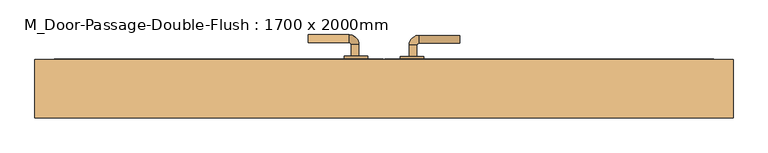
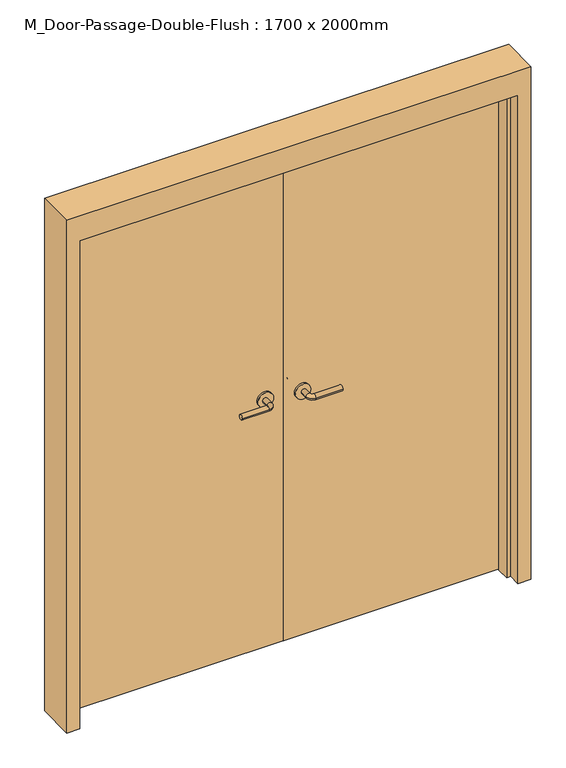
"""IFC4 building model written with IfcOpenShell, lengths in millimetres: door geometry, M_Door-Passage-Double-Flush : 1700 x 2000mm."""

from ifc_helpers import new_model, si_unit, point, frame, frame_2d, origin, origin_with_axes, place, context, project, spatial, polyline, circle_curve, ellipse_curve, trimmed, segment, composite_curve, outline, extrude, faceted_brep, source, transform, mapped, element, save
from ifc_brep_helpers import plane_surface, cylinder_surface, revolved_surface, advanced_brep


def m_door_passage_double_flush_1700_x_2000mm_c1a7d930(model_context):
    return source(origin(), model_context, "Body", "SolidModel", [
        advanced_brep(
        [(-65.009375, 28.35, 1016.0), (-85.009375, 28.35, 1016.0), (-65.009375, -1.65, 1016.0), (-85.009375, -1.65, 1016.0), (-90.009375, -6.65, 1016.0), (-90.009375, -26.65, 1016.0), (-195.009375, -26.65, 1016.0), (-195.009375, -6.65, 1016.0)],
        [
            (0, 1, circle_curve(frame((-75.009375, 28.35, 1016.0), z_axis=(0.0, 1.0, 0.0), x_axis=(-1.0, 0.0, 0.0)), 10.0)),
            (1, 0, circle_curve(frame((-75.009375, 28.35, 1016.0), z_axis=(0.0, 1.0, 0.0), x_axis=(-1.0, 0.0, 0.0)), 10.0)),
            (0, 2),
            (2, 3, circle_curve(frame((-75.009375, -1.65, 1016.0), z_axis=(0.0, 1.0, 0.0), x_axis=(-1.0, 0.0, 0.0)), 10.0)),
            (3, 1),
            (3, 2, circle_curve(frame((-75.009375, -1.65, 1016.0), z_axis=(0.0, 1.0, 0.0), x_axis=(-1.0, 0.0, 0.0)), 10.0)),
            (4, 3, circle_curve(frame((-90.009375, -1.65, 1016.0), z_axis=(0.0, 0.0, 1.0), x_axis=(1.0, 0.0, 0.0)), 5.0)),
            (2, 5, circle_curve(frame((-90.009375, -1.65, 1016.0), z_axis=(0.0, 0.0, -1.0), x_axis=(1.0, 0.0, 0.0)), 25.0)),
            (5, 4, circle_curve(frame((-90.009375, -16.65, 1016.0), z_axis=(1.0, 0.0, 0.0), x_axis=(0.0, 1.0, 0.0)), 10.0)),
            (4, 5, circle_curve(frame((-90.009375, -16.65, 1016.0), z_axis=(1.0, 0.0, 0.0), x_axis=(0.0, 1.0, 0.0)), 10.0)),
            (6, 7, circle_curve(frame((-195.009375, -16.65, 1016.0), z_axis=(-1.0, 0.0, 0.0), x_axis=(0.0, 1.0, 0.0)), 10.0)),
            (7, 6, circle_curve(frame((-195.009375, -16.65, 1016.0), z_axis=(-1.0, 0.0, 0.0), x_axis=(0.0, 1.0, 0.0)), 10.0)),
            (5, 6),
            (7, 4),
        ],
        [
            plane_surface(frame((-75.009375, 28.35, 1016.0), z_axis=(0.0, 1.0, 0.0), x_axis=(0.0, 0.0, 1.0))),
            cylinder_surface(frame((-75.009375, 28.35, 1016.0), z_axis=(0.0, 1.0, 0.0), x_axis=(-1.0, 0.0, 0.0)), 10.0),
            revolved_surface(trimmed(ellipse_curve(frame((-75.009375, -1.65, 1016.0), z_axis=(0.0, 1.0, 0.0), x_axis=(-1.0, 0.0, 0.0)), 10.0, 10.0), [point((-65.009375, -1.65, 1016.0))], [point((-85.009375, -1.65, 1016.0))], True, "CARTESIAN"), (-90.009375, -1.65, 1016.0), (0.0, 0.0, -1.0)),
            revolved_surface(trimmed(ellipse_curve(frame((-75.009375, -1.65, 1016.0), z_axis=(0.0, 1.0, 0.0), x_axis=(-1.0, 0.0, 0.0)), 10.0, 10.0), [point((-85.009375, -1.65, 1016.0))], [point((-65.009375, -1.65, 1016.0))], True, "CARTESIAN"), (-90.009375, -1.65, 1016.0), (0.0, 0.0, -1.0)),
            plane_surface(frame((-195.009375, -16.65, 1016.0), z_axis=(-1.0, 0.0, 0.0), x_axis=(0.0, 0.0, 1.0))),
            cylinder_surface(frame((-90.009375, -16.65, 1016.0), z_axis=(1.0, 0.0, 0.0), x_axis=(0.0, 1.0, 0.0)), 10.0),
        ],
        [
            (0, [[1, 2]]),
            (1, [[-1, 3, 4, 5]]),
            (1, [[-2, -5, 6, -3]]),
            (2, [[7, -4, 8, 9]]),
            (3, [[-8, -6, -7, 10]]),
            (4, [[11, 12]]),
            (5, [[-9, 13, -12, 14]]),
            (5, [[-10, -14, -11, -13]]),
        ],
    ),
        extrude(outline(composite_curve([segment(trimmed(circle_curve(frame_2d((1016.0, -72.509375)), 30.0), [point((1016.0, -42.509375))], [point((1016.0, -102.509375))], False, "CARTESIAN"), True, "CONTINUOUS"), segment(trimmed(circle_curve(frame_2d((1016.0, -72.509375)), 30.0), [point((1016.0, -102.509375))], [point((1016.0, -42.509375))], False, "CARTESIAN"), True, "CONTINUOUS")], self_intersect=False)), frame((0.0, 28.35, 0.0), z_axis=(0.0, 1.0, 0.0), x_axis=(0.0, 0.0, 1.0)), (0.0, 0.0, 1.0), 8.0),
        advanced_brep(
        [(-65.009375, 90.95, 1000.0), (-85.009375, 90.95, 1000.0), (-85.009375, 120.95, 1000.0), (-65.009375, 120.95, 1000.0), (-90.009375, 125.95, 1000.0), (-90.009375, 145.95, 1000.0), (-195.009375, 145.95, 1000.0), (-195.009375, 125.95, 1000.0)],
        [
            (0, 1, circle_curve(frame((-75.009375, 90.95, 1000.0), z_axis=(0.0, -1.0, 0.0), x_axis=(-1.0, 0.0, 0.0)), 10.0)),
            (1, 0, circle_curve(frame((-75.009375, 90.95, 1000.0), z_axis=(0.0, -1.0, 0.0), x_axis=(-1.0, 0.0, 0.0)), 10.0)),
            (1, 2),
            (2, 3, circle_curve(frame((-75.009375, 120.95, 1000.0), z_axis=(0.0, -1.0, 0.0), x_axis=(-1.0, 0.0, 0.0)), 10.0)),
            (3, 0),
            (3, 2, circle_curve(frame((-75.009375, 120.95, 1000.0), z_axis=(0.0, -1.0, 0.0), x_axis=(-1.0, 0.0, 0.0)), 10.0)),
            (4, 5, circle_curve(frame((-90.009375, 135.95, 1000.0), z_axis=(1.0, 0.0, 0.0), x_axis=(0.0, -1.0, 0.0)), 10.0)),
            (5, 3, circle_curve(frame((-90.009375, 120.95, 1000.0), z_axis=(0.0, 0.0, -1.0), x_axis=(1.0, 0.0, 0.0)), 25.0)),
            (2, 4, circle_curve(frame((-90.009375, 120.95, 1000.0), z_axis=(0.0, 0.0, 1.0), x_axis=(1.0, 0.0, 0.0)), 5.0)),
            (5, 4, circle_curve(frame((-90.009375, 135.95, 1000.0), z_axis=(1.0, 0.0, 0.0), x_axis=(0.0, -1.0, 0.0)), 10.0)),
            (6, 7, circle_curve(frame((-195.009375, 135.95, 1000.0), z_axis=(-1.0, 0.0, 0.0), x_axis=(0.0, -1.0, 0.0)), 10.0)),
            (7, 6, circle_curve(frame((-195.009375, 135.95, 1000.0), z_axis=(-1.0, 0.0, 0.0), x_axis=(0.0, -1.0, 0.0)), 10.0)),
            (4, 7),
            (6, 5),
        ],
        [
            plane_surface(frame((-75.009375, 90.95, 1000.0), z_axis=(0.0, -1.0, 0.0), x_axis=(0.0, 0.0, 1.0))),
            cylinder_surface(frame((-75.009375, 90.95, 1000.0), z_axis=(0.0, -1.0, 0.0), x_axis=(-1.0, 0.0, 0.0)), 10.0),
            revolved_surface(trimmed(ellipse_curve(frame((-75.009375, 120.95, 1000.0), z_axis=(0.0, 1.0, 0.0), x_axis=(-1.0, 0.0, 0.0)), 10.0, 10.0), [point((-65.009375, 120.95, 1000.0))], [point((-85.009375, 120.95, 1000.0))], True, "CARTESIAN"), (-90.009375, 120.95, 1000.0), (0.0, 0.0, -1.0)),
            revolved_surface(trimmed(ellipse_curve(frame((-75.009375, 120.95, 1000.0), z_axis=(0.0, 1.0, 0.0), x_axis=(-1.0, 0.0, 0.0)), 10.0, 10.0), [point((-85.009375, 120.95, 1000.0))], [point((-65.009375, 120.95, 1000.0))], True, "CARTESIAN"), (-90.009375, 120.95, 1000.0), (0.0, 0.0, -1.0)),
            plane_surface(frame((-195.009375, 135.95, 1000.0), z_axis=(-1.0, 0.0, 0.0), x_axis=(0.0, 0.0, 1.0))),
            cylinder_surface(frame((-90.009375, 135.95, 1000.0), z_axis=(1.0, 0.0, 0.0), x_axis=(0.0, -1.0, 0.0)), 10.0),
        ],
        [
            (0, [[1, 2]]),
            (1, [[3, 4, 5, -2]]),
            (1, [[-5, 6, -3, -1]]),
            (2, [[7, 8, -4, 9]]),
            (3, [[10, -9, -6, -8]]),
            (4, [[11, 12]]),
            (5, [[13, -11, 14, -7]]),
            (5, [[-14, -12, -13, -10]]),
        ],
    ),
        extrude(outline(composite_curve([segment(trimmed(circle_curve(frame_2d((1000.0, -72.509375)), 30.0), [point((1000.0, -42.509375))], [point((1000.0, -102.509375))], False, "CARTESIAN"), True, "CONTINUOUS"), segment(trimmed(circle_curve(frame_2d((1000.0, -72.509375)), 30.0), [point((1000.0, -102.509375))], [point((1000.0, -42.509375))], False, "CARTESIAN"), True, "CONTINUOUS")], self_intersect=False)), frame((0.0, 82.95, 0.0), z_axis=(0.0, 1.0, 0.0), x_axis=(0.0, 0.0, 1.0)), (0.0, 0.0, 1.0), 8.0),
        advanced_brep(
        [(65.009375, 28.35, 1000.0), (85.009375, 28.35, 1000.0), (85.009375, -1.65, 1000.0), (65.009375, -1.65, 1000.0), (90.009375, -6.65, 1000.0), (90.009375, -26.65, 1000.0), (195.009375, -26.65, 1000.0), (195.009375, -6.65, 1000.0)],
        [
            (0, 1, circle_curve(frame((75.009375, 28.35, 1000.0), z_axis=(0.0, 1.0, 0.0), x_axis=(1.0, 0.0, 0.0)), 10.0)),
            (1, 0, circle_curve(frame((75.009375, 28.35, 1000.0), z_axis=(0.0, 1.0, 0.0), x_axis=(1.0, 0.0, 0.0)), 10.0)),
            (1, 2),
            (2, 3, circle_curve(frame((75.009375, -1.65, 1000.0), z_axis=(0.0, 1.0, 0.0), x_axis=(1.0, 0.0, 0.0)), 10.0)),
            (3, 0),
            (3, 2, circle_curve(frame((75.009375, -1.65, 1000.0), z_axis=(0.0, 1.0, 0.0), x_axis=(1.0, 0.0, 0.0)), 10.0)),
            (4, 5, circle_curve(frame((90.009375, -16.65, 1000.0), z_axis=(-1.0, 0.0, 0.0), x_axis=(0.0, 1.0, 0.0)), 10.0)),
            (5, 3, circle_curve(frame((90.009375, -1.65, 1000.0), z_axis=(0.0, 0.0, -1.0), x_axis=(-1.0, 0.0, 0.0)), 25.0)),
            (2, 4, circle_curve(frame((90.009375, -1.65, 1000.0), z_axis=(0.0, 0.0, 1.0), x_axis=(-1.0, 0.0, 0.0)), 5.0)),
            (5, 4, circle_curve(frame((90.009375, -16.65, 1000.0), z_axis=(-1.0, 0.0, 0.0), x_axis=(0.0, 1.0, 0.0)), 10.0)),
            (6, 7, circle_curve(frame((195.009375, -16.65, 1000.0), z_axis=(1.0, 0.0, 0.0), x_axis=(0.0, 1.0, 0.0)), 10.0)),
            (7, 6, circle_curve(frame((195.009375, -16.65, 1000.0), z_axis=(1.0, 0.0, 0.0), x_axis=(0.0, 1.0, 0.0)), 10.0)),
            (4, 7),
            (6, 5),
        ],
        [
            plane_surface(frame((75.009375, 28.35, 1000.0), z_axis=(0.0, 1.0, 0.0), x_axis=(0.0, 0.0, 1.0))),
            cylinder_surface(frame((75.009375, 28.35, 1000.0), z_axis=(0.0, 1.0, 0.0), x_axis=(1.0, 0.0, 0.0)), 10.0),
            revolved_surface(trimmed(ellipse_curve(frame((75.009375, -1.65, 1000.0), z_axis=(0.0, -1.0, 0.0), x_axis=(1.0, 0.0, 0.0)), 10.0, 10.0), [point((65.009375, -1.65, 1000.0))], [point((85.009375, -1.65, 1000.0))], True, "CARTESIAN"), (90.009375, -1.65, 1000.0), (0.0, 0.0, -1.0)),
            revolved_surface(trimmed(ellipse_curve(frame((75.009375, -1.65, 1000.0), z_axis=(0.0, -1.0, 0.0), x_axis=(1.0, 0.0, 0.0)), 10.0, 10.0), [point((85.009375, -1.65, 1000.0))], [point((65.009375, -1.65, 1000.0))], True, "CARTESIAN"), (90.009375, -1.65, 1000.0), (0.0, 0.0, -1.0)),
            plane_surface(frame((195.009375, -16.65, 1000.0), z_axis=(1.0, 0.0, 0.0), x_axis=(0.0, 0.0, 1.0))),
            cylinder_surface(frame((90.009375, -16.65, 1000.0), z_axis=(-1.0, 0.0, 0.0), x_axis=(0.0, 1.0, 0.0)), 10.0),
        ],
        [
            (0, [[1, 2]]),
            (1, [[3, 4, 5, -2]]),
            (1, [[-5, 6, -3, -1]]),
            (2, [[7, 8, -4, 9]]),
            (3, [[10, -9, -6, -8]]),
            (4, [[11, 12]]),
            (5, [[13, -11, 14, -7]]),
            (5, [[-14, -12, -13, -10]]),
        ],
    ),
        extrude(outline(composite_curve([segment(trimmed(circle_curve(frame_2d((1000.0, 72.509375)), 30.0), [point((1000.0, 42.509375))], [point((1000.0, 102.509375))], False, "CARTESIAN"), True, "CONTINUOUS"), segment(trimmed(circle_curve(frame_2d((1000.0, 72.509375)), 30.0), [point((1000.0, 102.509375))], [point((1000.0, 42.509375))], False, "CARTESIAN"), True, "CONTINUOUS")], self_intersect=False)), frame((0.0, 28.35, 0.0), z_axis=(0.0, 1.0, 0.0), x_axis=(0.0, 0.0, 1.0)), (0.0, 0.0, 1.0), 8.0),
        advanced_brep(
        [(65.009375, 89.35, 1000.0), (85.009375, 89.35, 1000.0), (65.009375, 119.35, 1000.0), (85.009375, 119.35, 1000.0), (90.009375, 124.35, 1000.0), (90.009375, 144.35, 1000.0), (195.009375, 144.35, 1000.0), (195.009375, 124.35, 1000.0)],
        [
            (0, 1, circle_curve(frame((75.009375, 89.35, 1000.0), z_axis=(0.0, -1.0, 0.0), x_axis=(1.0, 0.0, 0.0)), 10.0)),
            (1, 0, circle_curve(frame((75.009375, 89.35, 1000.0), z_axis=(0.0, -1.0, 0.0), x_axis=(1.0, 0.0, 0.0)), 10.0)),
            (0, 2),
            (2, 3, circle_curve(frame((75.009375, 119.35, 1000.0), z_axis=(0.0, -1.0, 0.0), x_axis=(1.0, 0.0, 0.0)), 10.0)),
            (3, 1),
            (3, 2, circle_curve(frame((75.009375, 119.35, 1000.0), z_axis=(0.0, -1.0, 0.0), x_axis=(1.0, 0.0, 0.0)), 10.0)),
            (4, 3, circle_curve(frame((90.009375, 119.35, 1000.0), z_axis=(0.0, 0.0, 1.0), x_axis=(-1.0, 0.0, 0.0)), 5.0)),
            (2, 5, circle_curve(frame((90.009375, 119.35, 1000.0), z_axis=(0.0, 0.0, -1.0), x_axis=(-1.0, 0.0, 0.0)), 25.0)),
            (5, 4, circle_curve(frame((90.009375, 134.35, 1000.0), z_axis=(-1.0, 0.0, 0.0), x_axis=(0.0, -1.0, 0.0)), 10.0)),
            (4, 5, circle_curve(frame((90.009375, 134.35, 1000.0), z_axis=(-1.0, 0.0, 0.0), x_axis=(0.0, -1.0, 0.0)), 10.0)),
            (6, 7, circle_curve(frame((195.009375, 134.35, 1000.0), z_axis=(1.0, 0.0, 0.0), x_axis=(0.0, -1.0, 0.0)), 10.0)),
            (7, 6, circle_curve(frame((195.009375, 134.35, 1000.0), z_axis=(1.0, 0.0, 0.0), x_axis=(0.0, -1.0, 0.0)), 10.0)),
            (5, 6),
            (7, 4),
        ],
        [
            plane_surface(frame((75.009375, 89.35, 1000.0), z_axis=(0.0, -1.0, 0.0), x_axis=(0.0, 0.0, 1.0))),
            cylinder_surface(frame((75.009375, 89.35, 1000.0), z_axis=(0.0, -1.0, 0.0), x_axis=(1.0, 0.0, 0.0)), 10.0),
            revolved_surface(trimmed(ellipse_curve(frame((75.009375, 119.35, 1000.0), z_axis=(0.0, -1.0, 0.0), x_axis=(1.0, 0.0, 0.0)), 10.0, 10.0), [point((65.009375, 119.35, 1000.0))], [point((85.009375, 119.35, 1000.0))], True, "CARTESIAN"), (90.009375, 119.35, 1000.0), (0.0, 0.0, -1.0)),
            revolved_surface(trimmed(ellipse_curve(frame((75.009375, 119.35, 1000.0), z_axis=(0.0, -1.0, 0.0), x_axis=(1.0, 0.0, 0.0)), 10.0, 10.0), [point((85.009375, 119.35, 1000.0))], [point((65.009375, 119.35, 1000.0))], True, "CARTESIAN"), (90.009375, 119.35, 1000.0), (0.0, 0.0, -1.0)),
            plane_surface(frame((195.009375, 134.35, 1000.0), z_axis=(1.0, 0.0, 0.0), x_axis=(0.0, 0.0, 1.0))),
            cylinder_surface(frame((90.009375, 134.35, 1000.0), z_axis=(-1.0, 0.0, 0.0), x_axis=(0.0, -1.0, 0.0)), 10.0),
        ],
        [
            (0, [[1, 2]]),
            (1, [[-1, 3, 4, 5]]),
            (1, [[-2, -5, 6, -3]]),
            (2, [[7, -4, 8, 9]]),
            (3, [[-8, -6, -7, 10]]),
            (4, [[11, 12]]),
            (5, [[-9, 13, -12, 14]]),
            (5, [[-10, -14, -11, -13]]),
        ],
    ),
        extrude(outline(composite_curve([segment(trimmed(circle_curve(frame_2d((1000.0, 72.509375)), 30.0), [point((1000.0, 42.509375))], [point((1000.0, 102.509375))], False, "CARTESIAN"), True, "CONTINUOUS"), segment(trimmed(circle_curve(frame_2d((1000.0, 72.509375)), 30.0), [point((1000.0, 102.509375))], [point((1000.0, 42.509375))], False, "CARTESIAN"), True, "CONTINUOUS")], self_intersect=False)), frame((0.0, 81.35, 0.0), z_axis=(0.0, 1.0, 0.0), x_axis=(0.0, 0.0, 1.0)), (0.0, 0.0, 1.0), 8.0),
        extrude(outline(polyline([(850.0, 36.35), (1.5875, 36.35), (1.5875, 82.95), (850.0, 82.95), (850.0, 36.35)])), origin_with_axes(), (0.0, 0.0, 1.0), 2000.0),
        extrude(outline(polyline([(-1.5875, 36.35), (-850.0, 36.35), (-850.0, 82.95), (-1.5875, 82.95), (-1.5875, 36.35)])), origin_with_axes(), (0.0, 0.0, 1.0), 2000.0),
        faceted_brep([(850.0, 31.5875, 0.0), (850.0, 81.35, 0.0), (900.0, 81.35, 0.0), (900.0, -68.65, 0.0), (850.0, -68.65, 0.0), (850.0, -19.4375, 0.0), (834.125, -19.4375, 0.0), (834.125, 31.5875, 0.0), (850.0, 31.5875, 2000.0), (850.0, 81.35, 2000.0), (-850.0, 81.35, 2000.0), (-850.0, 81.35, 0.0), (-900.0, 81.35, 0.0), (-900.0, 81.35, 2100.0), (900.0, 81.35, 2100.0), (900.0, -68.65, 2100.0), (-900.0, -68.65, 2100.0), (-900.0, -68.65, 0.0), (-850.0, -68.65, 0.0), (-850.0, -68.65, 2000.0), (850.0, -68.65, 2000.0), (850.0, -19.4375, 2000.0), (-850.0, -19.4375, 2000.0), (-850.0, -19.4375, 0.0), (-834.125, -19.4375, 0.0), (-834.125, -19.4375, 1984.125), (834.125, -19.4375, 1984.125), (834.125, 31.5875, 1984.125), (-834.125, 31.5875, 1984.125), (-834.125, 31.5875, 0.0), (-850.0, 31.5875, 0.0), (-850.0, 31.5875, 2000.0)], [[[0, 1, 2, 3, 4, 5, 6, 7]], [[1, 0, 8, 9]], [[2, 1, 9, 10, 11, 12, 13, 14]], [[3, 2, 14, 15]], [[4, 3, 15, 16, 17, 18, 19, 20]], [[5, 4, 20, 21]], [[6, 5, 21, 22, 23, 24, 25, 26]], [[7, 6, 26, 27]], [[0, 7, 27, 28, 29, 30, 31, 8]], [[9, 8, 31, 10]], [[20, 19, 22, 21]], [[26, 25, 28, 27]], [[12, 11, 30, 29, 24, 23, 18, 17]], [[11, 10, 31, 30]], [[13, 12, 17, 16]], [[19, 18, 23, 22]], [[25, 24, 29, 28]], [[15, 14, 13, 16]]]),
    ])


if __name__ == "__main__":
    model = new_model("IFC4")
    model_context = context("Model", 3, world=origin())
    ifc_project = project(units=[si_unit("LENGTHUNIT", "METRE", prefix="MILLI")], contexts=[model_context])
    site = spatial("IfcSite", under=ifc_project)
    building = spatial("IfcBuilding", under=site)
    placement = place(None, origin())
    m_door_passage_double_flush_1700_x_2000mm_shape = m_door_passage_double_flush_1700_x_2000mm_c1a7d930(model_context)
    element("IfcDoor", 1, ObjectType="M_Door-Passage-Double-Flush : 1700 x 2000mm", at=placement, inside=building, context=model_context, shape_type="MappedRepresentation", body=[
        mapped(m_door_passage_double_flush_1700_x_2000mm_shape, transform((0.0, 0.0, 0.0), x_axis=(1.0, 0.0, 0.0), y_axis=(0.0, 1.0, 0.0), z_axis=(0.0, 0.0, 1.0))),
    ])
    save(model, "model.ifc")

# Revit data of these elements
# Type "M_Door-Passage-Double-Flush : 1700 x 2000mm"
#   Type Mark = "31"
#   Analytic Construction = "Metal"
#   Thickness = 45 mm
#   Thermal Resistance (R) = 0.270118 (m²·K)/W
#   Swing Angle [instance default] = 90.00°
#   Strike Height = 1000 mm
#   SinglePanelWidth = 850 mm
#   Rough Width [instance default] = 1800 mm
#   Rough Height [instance default] = 2100 mm
#   MFOpeningHeight [instance default] = 100 mm
#   MFOpeningWidth [instance default] = 100 mm
#   Inset Calculate [instance default] = 105 mm
#   Masonry Inset [instance default] = 25 mm
#   Height = 2000 mm
#   Width = 1700 mm
#   Heat Transfer Coefficient (U) = 3.70223 W/(m²·K)
#   Masonry Frame Depth = 150 mm
#   Masonry Frame [instance default] = yes
#   Function = 1
#   Dry Wall Frame [instance default] = no
#   Panel Material = Metal Door - Brindle
#   Frame Material = Metal - Painted - Grey
#   Door Handle Material = Aluminum
#   Visual Light Transmittance = 0
#   Solar Heat Gain Coefficient = 0
#   Wall Closure = (empty or 0)
# Element 1 (IfcDoor, "M_Door-Passage-Double-Flush : 1700 x 2000mm")
#   Materials on its faces: "Aluminum", "Metal - Painted - Grey", "Metal Door - Brindle"
# Materials
#   "Metal Door - Brindle": class "Paint", colour RGB 164 133 98, transparency 0
#   "Metal - Painted - Grey": class "Paint", colour RGB 104 104 104, transparency 0
#   "Aluminum": class "Metal", colour RGB 244 245 246, transparency 0, Description = "Aluminum 6061", Cost = 0
